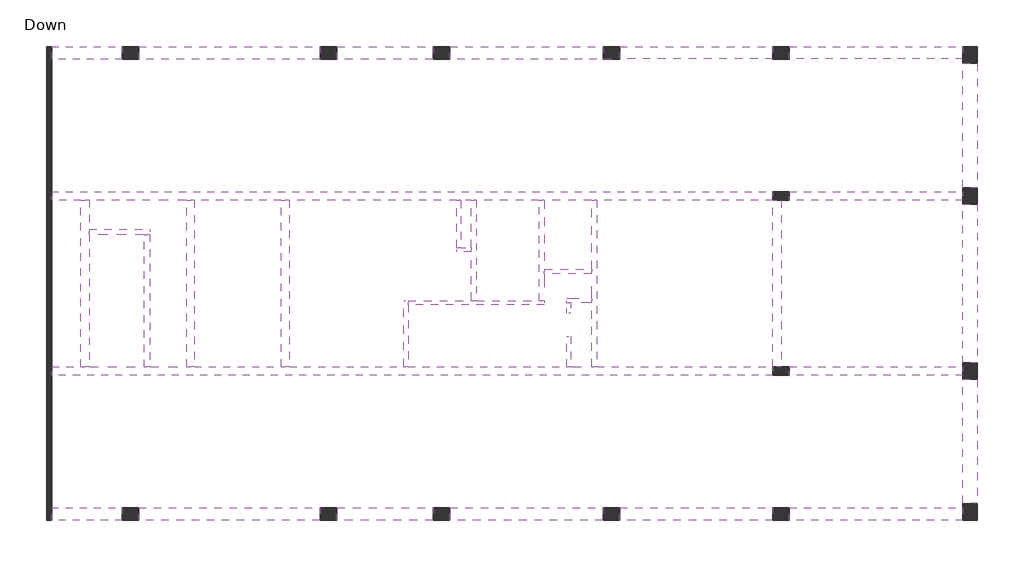
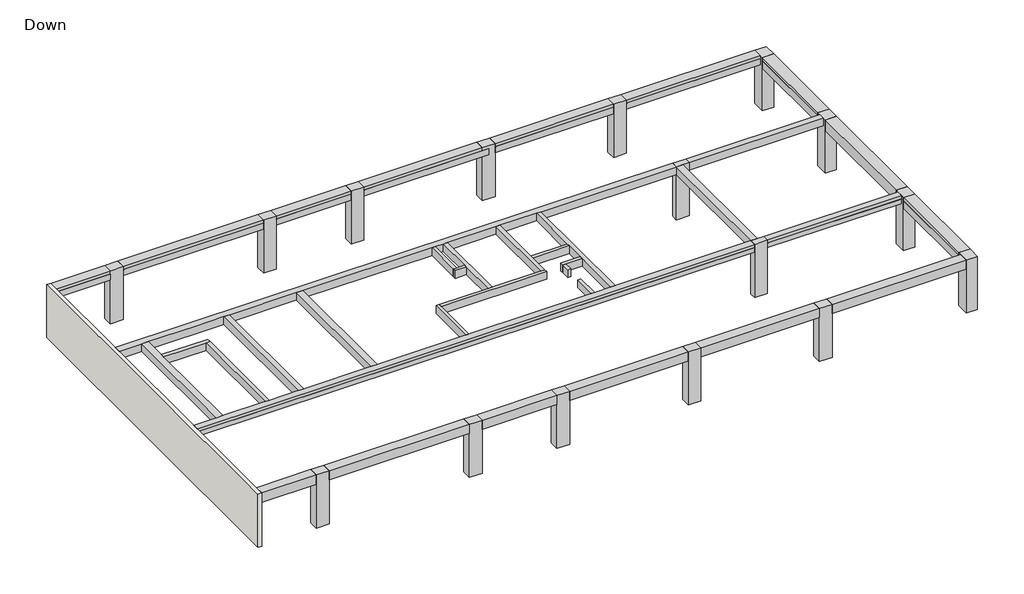
# One storey: 36 beams, 16 columns, 1 wall.
"""IFC4 building model written with IfcOpenShell, lengths in millimetres."""

from ifc_helpers import new_model, si_unit, frame, origin, place, context, project, spatial, polyline, outline, extrude, faceted_brep, element, save

model = new_model("IFC4")

# Units and contexts
model_context = context("Model", 3, world=origin())
ifc_project = project(units=[si_unit("LENGTHUNIT", "METRE", prefix="MILLI")], contexts=[model_context])

# Site, building, storey
site = spatial("IfcSite", under=ifc_project)
building = spatial("IfcBuilding", under=site)
storey = spatial("IfcBuildingStorey", under=building, Name="Down", Elevation=0.0)

# Beams
placement = place(None, origin())
element("IfcBeam", 1, ObjectType="Concrete Rectengular Beam : 20/50", at=placement, inside=storey, context=model_context, shape_type="Brep", body=[
    faceted_brep([(-13392.6687444, -4379.553058, 3500.0), (-13192.6687444, -4379.553058, 3500.0), (-13192.6687444, -1379.553058, 3500.0), (-13192.6687444, -1179.553058, 3500.0), (-13392.6687444, -1179.553058, 3500.0), (-13192.6687444, -4379.553058, 3300.0), (-13192.6687444, -4379.553058, 3000.0), (-13192.6687444, -1379.553058, 3000.0), (-13192.6687444, -1179.553058, 3000.0), (-13192.6687444, -1179.553058, 3300.0), (-13392.6687444, -4379.553058, 3000.0), (-13392.6687444, -1179.553058, 3000.0), (-13392.6687444, -1179.553058, 3300.0), (-13392.6687444, -4379.553058, 3300.0)], [[[0, 1, 2, 3, 4]], [[1, 5, 6, 7, 8, 9, 3, 2]], [[6, 10, 11, 8, 7]], [[0, 4, 12, 11, 10, 13]], [[1, 0, 13, 10, 6, 5]], [[4, 3, 9, 8, 11, 12]]]),
])
element("IfcBeam", 2, ObjectType="Concrete Rectengular Beam : 20/50", at=placement, inside=storey, context=model_context, shape_type="Brep", body=[
    faceted_brep([(-13192.6687444, -1179.553058, 3500.0), (-13192.6687444, -1379.553058, 3500.0), (-6622.8724137, -1379.553058, 3500.0), (-6622.8724137, -1179.553058, 3500.0), (-6872.8724137, -1179.553058, 3500.0), (-9902.8742387, -1179.553058, 3500.0), (-10152.8742387, -1179.553058, 3500.0), (-13192.6687444, -1379.553058, 3300.0), (-13192.6687444, -1379.553058, 3000.0), (-6622.8724137, -1379.553058, 3000.0), (-6622.8724137, -1379.553058, 3300.0), (-13192.6687444, -1179.553058, 3000.0), (-10152.8742387, -1179.553058, 3000.0), (-9902.8742387, -1179.553058, 3000.0), (-6872.8724137, -1179.553058, 3000.0), (-6622.8724137, -1179.553058, 3000.0), (-13192.6687444, -1179.553058, 3300.0), (-6622.8724137, -1179.553058, 3300.0)], [[[0, 1, 2, 3, 4, 5, 6]], [[2, 1, 7, 8, 9, 10]], [[8, 11, 12, 13, 14, 15, 9]], [[15, 14, 13, 12, 11, 16, 0, 6, 5, 4, 3, 17]], [[1, 0, 16, 11, 8, 7]], [[3, 2, 10, 9, 15, 17]]]),
])
element("IfcBeam", 3, ObjectType="Concrete Rectengular Beam : 20/50", at=placement, inside=storey, context=model_context, shape_type="Brep", body=[
    faceted_brep([(-10152.8742387, 1160.4573545, 3500.0), (-10152.8742387, 1360.4573545, 3500.0), (-10647.8742387, 1360.4573545, 3500.0), (-10847.8742387, 1360.4573545, 3500.0), (-10847.8742387, 1160.4573545, 3500.0), (-10152.8742387, 1360.4573545, 3300.0), (-10152.8742387, 1360.4573545, 3000.0), (-10647.8742387, 1360.4573545, 3000.0), (-10847.8742387, 1360.4573545, 3000.0), (-10847.8742387, 1360.4573545, 3300.0), (-10152.8742387, 1160.4573545, 3000.0), (-10847.8742387, 1160.4573545, 3000.0), (-10847.8742387, 1160.4573545, 3300.0), (-10152.8742387, 1160.4573545, 3300.0)], [[[0, 1, 2, 3, 4]], [[1, 5, 6, 7, 8, 9, 3, 2]], [[6, 10, 11, 8, 7]], [[0, 4, 12, 11, 10, 13]], [[1, 0, 13, 10, 6, 5]], [[4, 3, 9, 8, 11, 12]]]),
])
element("IfcBeam", 4, ObjectType="Concrete Rectengular Beam : 20/50", at=placement, inside=storey, context=model_context, shape_type="Brep", body=[
    faceted_brep([(-10847.8742387, 1360.4573545, 3500.0), (-10647.8742387, 1360.4573545, 3500.0), (-10647.8742387, 3660.4573545, 3500.0), (-10847.8742387, 3660.4573545, 3500.0), (-10647.8742387, 1360.4573545, 3300.0), (-10647.8742387, 1360.4573545, 3000.0), (-10647.8742387, 3660.4573545, 3000.0), (-10647.8742387, 3660.4573545, 3300.0), (-10847.8742387, 1360.4573545, 3000.0), (-10847.8742387, 3660.4573545, 3000.0), (-10847.8742387, 3660.4573545, 3300.0), (-10847.8742387, 1360.4573545, 3300.0)], [[[0, 1, 2, 3]], [[1, 4, 5, 6, 7, 2]], [[5, 8, 9, 6]], [[0, 3, 10, 9, 8, 11]], [[1, 0, 11, 8, 5, 4]], [[3, 2, 7, 6, 9, 10]]]),
])
element("IfcBeam", 5, ObjectType="Concrete Rectengular Beam : 20/50", at=placement, inside=storey, context=model_context, shape_type="Brep", body=[
    faceted_brep([(-5552.8714262, -2899.5501705, 3500.0), (-5352.8714262, -2899.5501705, 3500.0), (-5352.8714262, -2899.5501705, 3300.0), (-5352.8714262, -2899.5501705, 3000.0), (-5552.8714262, -2899.5501705, 3000.0), (-5552.8714262, -2899.5501705, 3300.0), (-5552.8714262, -4379.553058, 3500.0), (-5352.8714262, -4379.553058, 3500.0), (-5352.8714262, -4379.553058, 3300.0), (-5352.8714262, -4379.553058, 3000.0), (-5552.8714262, -4379.553058, 3000.0), (-5552.8714262, -4379.553058, 3300.0)], [[[0, 1, 2, 3, 4, 5]], [[1, 0, 6, 7]], [[1, 7, 8, 9, 3, 2]], [[4, 3, 9, 10]], [[6, 0, 5, 4, 10, 11]], [[7, 6, 11, 10, 9, 8]]]),
])
element("IfcBeam", 6, ObjectType="Concrete Rectengular Beam : 20/50", at=placement, inside=storey, context=model_context, shape_type="Brep", body=[
    faceted_brep([(-4337.2434753, -1279.553058, 3500.0), (-4337.2434753, -1079.553058, 3500.0), (-5552.8714262, -1079.553058, 3500.0), (-5552.8714262, -1279.553058, 3500.0), (-5352.8714262, -1279.553058, 3500.0), (-4337.2434753, -1079.553058, 3300.0), (-4337.2434753, -1079.553058, 3000.0), (-5552.8714262, -1079.553058, 3000.0), (-5552.8714262, -1079.553058, 3300.0), (-4337.2434753, -1279.553058, 3000.0), (-5352.8714262, -1279.553058, 3000.0), (-5552.8714262, -1279.553058, 3000.0), (-4337.2434753, -1279.553058, 3300.0), (-5552.8714262, -1279.553058, 3300.0)], [[[0, 1, 2, 3, 4]], [[2, 1, 5, 6, 7, 8]], [[6, 9, 10, 11, 7]], [[11, 10, 9, 12, 0, 4, 3, 13]], [[1, 0, 12, 9, 6, 5]], [[3, 2, 8, 7, 11, 13]]]),
])
element("IfcBeam", 7, ObjectType="Concrete Rectengular Beam : 20/50", at=placement, inside=storey, context=model_context, shape_type="Brep", body=[
    faceted_brep([(-5352.8714262, -1799.553058, 3500.0), (-5552.8714262, -1799.553058, 3500.0), (-5552.8714262, -1799.553058, 3300.0), (-5552.8714262, -1799.553058, 3000.0), (-5352.8714262, -1799.553058, 3000.0), (-5352.8714262, -1799.553058, 3300.0), (-5352.8714262, -1279.553058, 3500.0), (-5552.8714262, -1279.553058, 3500.0), (-5552.8714262, -1279.553058, 3300.0), (-5552.8714262, -1279.553058, 3000.0), (-5352.8714262, -1279.553058, 3000.0), (-5352.8714262, -1279.553058, 3300.0)], [[[0, 1, 2, 3, 4, 5]], [[1, 0, 6, 7]], [[1, 7, 8, 9, 3, 2]], [[4, 3, 9, 10]], [[6, 0, 5, 4, 10, 11]], [[7, 6, 11, 10, 9, 8]]]),
])
element("IfcBeam", 8, ObjectType="Concrete Rectengular Beam : 20/50", at=placement, inside=storey, context=model_context, shape_type="Brep", body=[
    faceted_brep([(-6622.8724137, 320.446942, 3500.0), (-6622.8724137, 120.446942, 3500.0), (-4337.2434753, 120.446942, 3500.0), (-4337.2434753, 320.446942, 3500.0), (-6622.8724137, 320.446942, 3000.0), (-6622.8724137, 320.446942, 3300.0), (-4337.2434753, 320.446942, 3300.0), (-4337.2434753, 320.446942, 3000.0), (-6622.8724137, 120.446942, 3000.0), (-4337.2434753, 120.446942, 3000.0), (-6622.8724137, 120.446942, 3300.0), (-4337.2434753, 120.446942, 3300.0)], [[[0, 1, 2, 3]], [[4, 5, 0, 3, 6, 7]], [[8, 4, 7, 9]], [[1, 10, 8, 9, 11, 2]], [[1, 0, 5, 4, 8, 10]], [[3, 2, 11, 9, 7, 6]]]),
])
element("IfcBeam", 9, ObjectType="Concrete Rectengular Beam : 25/50", at=placement, inside=storey, context=model_context, shape_type="Brep", body=[
    faceted_brep([(-25647.8929888, 2002.2215378, 3500.0), (-25647.8929888, 2252.2215378, 3500.0), (-28552.8929888, 2252.2215378, 3500.0), (-28552.8929888, 2002.2215378, 3500.0), (-25897.8929888, 2002.2215378, 3500.0), (-25647.8929888, 2002.2215378, 3000.0), (-28552.8929888, 2002.2215378, 3000.0), (-25897.8929888, 2002.2215378, 3000.0), (-25647.8929888, 2252.2215378, 3000.0), (-28552.8929888, 2252.2215378, 3000.0)], [[[0, 1, 2, 3, 4]], [[5, 0, 4, 3, 6, 7]], [[8, 5, 7, 6, 9]], [[1, 8, 9, 2]], [[3, 2, 9, 6]], [[1, 0, 5, 8]]]),
])
element("IfcBeam", 10, ObjectType="Concrete Rectengular Beam : 25/50", at=placement, inside=storey, context=model_context, shape_type="Brep", body=[
    faceted_brep([(-25647.8929888, 2002.2215378, 3500.0), (-25897.8929888, 2002.2215378, 3500.0), (-25897.8929888, -4379.553058, 3500.0), (-25647.8929888, -4379.553058, 3500.0), (-25897.8929888, 2002.2215378, 3000.0), (-25897.8929888, -4379.553058, 3000.0), (-25647.8929888, 2002.2215378, 3000.0), (-25647.8929888, -4379.553058, 3000.0), (-25647.8929888, -4379.553058, 3300.0)], [[[0, 1, 2, 3]], [[1, 4, 5, 2]], [[4, 6, 7, 5]], [[6, 0, 3, 8, 7]], [[1, 0, 6, 4]], [[3, 2, 5, 7, 8]]]),
])
element("IfcBeam", 11, ObjectType="Concrete Rectengular Beam : 25/50", at=placement, inside=storey, context=model_context, shape_type="Brep", body=[
    faceted_brep([(-9902.8742387, 3660.4573545, 3500.0), (-10152.8742387, 3660.4573545, 3500.0), (-10152.8742387, 1360.4573545, 3500.0), (-10152.8742387, 1160.4573545, 3500.0), (-10152.8742387, -1179.553058, 3500.0), (-9902.8742387, -1179.553058, 3500.0), (-9902.8742387, 3660.4573545, 3000.0), (-9902.8742387, 3660.4573545, 3300.0), (-9902.8742387, -1179.553058, 3300.0), (-9902.8742387, -1179.553058, 3000.0), (-10152.8742387, 3660.4573545, 3000.0), (-10152.8742387, -1179.553058, 3000.0), (-10152.8742387, 1160.4573545, 3000.0), (-10152.8742387, 1360.4573545, 3000.0), (-10152.8742387, 3660.4573545, 3300.0), (-10152.8742387, -1179.553058, 3300.0)], [[[0, 1, 2, 3, 4, 5]], [[6, 7, 0, 5, 8, 9]], [[10, 6, 9, 11, 12, 13]], [[1, 14, 10, 13, 12, 11, 15, 4, 3, 2]], [[1, 0, 7, 6, 10, 14]], [[5, 4, 15, 11, 9, 8]]]),
])
element("IfcBeam", 12, ObjectType="Concrete Rectengular Beam : 25/50", at=placement, inside=storey, context=model_context, shape_type="Brep", body=[
    faceted_brep([(-6622.8724137, 3660.4573545, 3500.0), (-6872.8724137, 3660.4573545, 3500.0), (-6872.8724137, -1179.553058, 3500.0), (-6622.8724137, -1179.553058, 3500.0), (-6622.8724137, 120.446942, 3500.0), (-6622.8724137, 320.446942, 3500.0), (-6622.8724137, 3660.4573545, 3000.0), (-6622.8724137, 3660.4573545, 3300.0), (-6622.8724137, -1179.553058, 3000.0), (-6622.8724137, 120.446942, 3000.0), (-6622.8724137, 320.446942, 3000.0), (-6872.8724137, 3660.4573545, 3000.0), (-6872.8724137, -1179.553058, 3000.0), (-6872.8724137, 3660.4573545, 3300.0), (-6872.8724137, -1179.553058, 3300.0)], [[[0, 1, 2, 3, 4, 5]], [[6, 7, 0, 5, 4, 3, 8, 9, 10]], [[11, 6, 10, 9, 8, 12]], [[1, 13, 11, 12, 14, 2]], [[1, 0, 7, 6, 11, 13]], [[3, 2, 14, 12, 8]]]),
])
element("IfcBeam", 13, ObjectType="Concrete Rectengular Beam : 25/50", at=placement, inside=storey, context=model_context, shape_type="Brep", body=[
    faceted_brep([(-4087.2434753, 3660.4573545, 3500.0), (-4337.2434753, 3660.4573545, 3500.0), (-4337.2434753, 320.446942, 3500.0), (-4337.2434753, 120.446942, 3500.0), (-4337.2434753, -1079.553058, 3500.0), (-4337.2434753, -1279.553058, 3500.0), (-4337.2434753, -4379.553058, 3500.0), (-4087.2434753, -4379.553058, 3500.0), (-4087.2434753, 3660.4573545, 3000.0), (-4087.2434753, 3660.4573545, 3300.0), (-4087.2434753, -4379.553058, 3300.0), (-4087.2434753, -4379.553058, 3000.0), (-4337.2434753, 3660.4573545, 3000.0), (-4337.2434753, -4379.553058, 3000.0), (-4337.2434753, -1279.553058, 3000.0), (-4337.2434753, -1079.553058, 3000.0), (-4337.2434753, 120.446942, 3000.0), (-4337.2434753, 320.446942, 3000.0), (-4337.2434753, 3660.4573545, 3300.0), (-4337.2434753, -4379.553058, 3300.0)], [[[0, 1, 2, 3, 4, 5, 6, 7]], [[8, 9, 0, 7, 10, 11]], [[12, 8, 11, 13, 14, 15, 16, 17]], [[1, 18, 12, 17, 16, 15, 14, 13, 19, 6, 5, 4, 3, 2]], [[1, 0, 9, 8, 12, 18]], [[7, 6, 19, 13, 11, 10]]]),
])
element("IfcBeam", 14, ObjectType="Concrete Rectengular Beam : 35/50", at=placement, inside=storey, context=model_context, shape_type="Brep", body=[
    faceted_brep([(-23497.8929888, 3660.4573545, 3500.0), (-23847.8929888, 3660.4573545, 3500.0), (-23847.8929888, -4379.553058, 3500.0), (-23497.8929888, -4379.553058, 3500.0), (-23497.8929888, 3660.4573545, 3000.0), (-23497.8929888, 3660.4573545, 3300.0), (-23497.8929888, -4379.553058, 3300.0), (-23497.8929888, -4379.553058, 3000.0), (-23847.8929888, 3660.4573545, 3000.0), (-23847.8929888, -4379.553058, 3000.0), (-23847.8929888, 3660.4573545, 3300.0), (-23847.8929888, -4379.553058, 3300.0)], [[[0, 1, 2, 3]], [[4, 5, 0, 3, 6, 7]], [[8, 4, 7, 9]], [[1, 10, 8, 9, 11, 2]], [[1, 0, 5, 4, 8, 10]], [[3, 2, 11, 9, 7, 6]]]),
])
element("IfcBeam", 15, ObjectType="Concrete Rectengular Beam : 40/50", at=placement, inside=storey, context=model_context, shape_type="Brep", body=[
    faceted_brep([(5187.1402675, 3660.4573545, 3500.0), (13547.1501363, 3660.4573545, 3500.0), (13547.1501363, 4055.4573545, 3500.0), (5187.1402675, 4055.4573545, 3500.0), (13547.1501363, 3660.4573545, 3000.0), (13547.1501363, 3660.4573545, 3300.0), (5187.1402675, 3660.4573545, 3000.0), (5187.1402675, 4060.4573545, 3000.0), (13547.1501363, 4060.4573545, 3000.0), (5187.1402675, 4060.4573545, 3300.0), (13547.1501363, 4060.4573545, 3300.0), (13547.1501363, 4055.4573545, 3300.0), (5187.1402675, 4055.4573545, 3300.0)], [[[0, 1, 2, 3]], [[4, 5, 1, 0, 6]], [[4, 6, 7, 8]], [[8, 7, 9, 10]], [[1, 5, 4, 8, 10, 11, 2]], [[6, 0, 3, 12, 9, 7]], [[12, 11, 10, 9]], [[11, 12, 3, 2]]]),
])
element("IfcBeam", 16, ObjectType="Concrete Rectengular Beam : 40/50", at=placement, inside=storey, context=model_context, shape_type="Brep", body=[
    faceted_brep([(13547.1501363, -4379.553058, 3500.0), (5187.1402675, -4379.553058, 3500.0), (5187.1402675, -4774.553058, 3500.0), (13547.1501363, -4774.553058, 3500.0), (5187.1402675, -4779.553058, 3000.0), (13547.1501363, -4779.553058, 3000.0), (13547.1501363, -4779.553058, 3300.0), (5187.1402675, -4779.553058, 3300.0), (13547.1501363, -4379.553058, 3000.0), (5187.1402675, -4379.553058, 3000.0), (13547.1501363, -4379.553058, 3300.0), (13547.1501363, -4774.553058, 3300.0), (5187.1402675, -4774.553058, 3300.0)], [[[0, 1, 2, 3]], [[4, 5, 6, 7]], [[8, 5, 4, 9]], [[0, 10, 8, 9, 1]], [[8, 10, 0, 3, 11, 6, 5]], [[9, 4, 7, 12, 2, 1]], [[11, 12, 7, 6]], [[12, 11, 3, 2]]]),
])
element("IfcBeam", 17, ObjectType="Concrete Rectengular Beam : 40/50", at=placement, inside=storey, context=model_context, shape_type="Brep", body=[
    faceted_brep([(4387.1402675, 3660.4573545, 3500.0), (4387.1402675, 4055.4573545, 3500.0), (-30362.89442, 4055.4573545, 3500.0), (-30362.89442, 3660.4573545, 3500.0), (-28952.8929888, 3660.4573545, 3500.0), (-28552.8929888, 3660.4573545, 3500.0), (-25647.8929888, 3660.4573545, 3500.0), (-23847.8929888, 3660.4573545, 3500.0), (-23497.8929888, 3660.4573545, 3500.0), (-19308.8564427, 3660.4573545, 3500.0), (-18908.8564427, 3660.4573545, 3500.0), (-10847.8742387, 3660.4573545, 3500.0), (-10647.8742387, 3660.4573545, 3500.0), (-10152.8742387, 3660.4573545, 3500.0), (-9902.8742387, 3660.4573545, 3500.0), (-6872.8724137, 3660.4573545, 3500.0), (-6622.8724137, 3660.4573545, 3500.0), (-4337.2434753, 3660.4573545, 3500.0), (-4087.2434753, 3660.4573545, 3500.0), (4387.1402675, 4060.4573545, 3300.0), (4387.1402675, 4060.4573545, 3000.0), (-30362.89442, 4060.4573545, 3000.0), (-30362.89442, 4060.4573545, 3300.0), (4387.1402675, 3660.4573545, 3000.0), (-4087.2434753, 3660.4573545, 3000.0), (-4337.2434753, 3660.4573545, 3000.0), (-6622.8724137, 3660.4573545, 3000.0), (-6872.8724137, 3660.4573545, 3000.0), (-9902.8742387, 3660.4573545, 3000.0), (-10152.8742387, 3660.4573545, 3000.0), (-10647.8742387, 3660.4573545, 3000.0), (-10847.8742387, 3660.4573545, 3000.0), (-18908.8564427, 3660.4573545, 3000.0), (-19308.8564427, 3660.4573545, 3000.0), (-23497.8929888, 3660.4573545, 3000.0), (-23847.8929888, 3660.4573545, 3000.0), (-28552.8929888, 3660.4573545, 3000.0), (-28952.8929888, 3660.4573545, 3000.0), (-30362.89442, 3660.4573545, 3000.0), (4387.1402675, 3660.4573545, 3300.0), (-30362.89442, 3660.4573545, 3300.0), (4387.1402675, 4055.4573545, 3300.0), (-30362.89442, 4055.4573545, 3300.0)], [[[0, 1, 2, 3, 4, 5, 6, 7, 8, 9, 10, 11, 12, 13, 14, 15, 16, 17, 18]], [[19, 20, 21, 22]], [[20, 23, 24, 25, 26, 27, 28, 29, 30, 31, 32, 33, 34, 35, 36, 37, 38, 21]], [[23, 39, 0, 18, 17, 16, 15, 14, 13, 12, 11, 10, 9, 8, 7, 6, 5, 4, 3, 40, 38, 37, 36, 35, 34, 33, 32, 31, 30, 29, 28, 27, 26, 25, 24]], [[23, 20, 19, 41, 1, 0, 39]], [[41, 19, 22, 42]], [[1, 41, 42, 2]], [[3, 2, 42, 22, 21, 38, 40]]]),
])
element("IfcBeam", 18, ObjectType="Concrete Rectengular Beam : 40/50", at=placement, inside=storey, context=model_context, shape_type="Brep", body=[
    faceted_brep([(4387.1402675, -4774.553058, 3500.0), (4387.1402675, -4379.553058, 3500.0), (-4087.2434753, -4379.553058, 3500.0), (-4337.2434753, -4379.553058, 3500.0), (-5352.8714262, -4379.553058, 3500.0), (-5552.8714262, -4379.553058, 3500.0), (-13192.6687444, -4379.553058, 3500.0), (-13392.6687444, -4379.553058, 3500.0), (-18908.8564427, -4379.553058, 3500.0), (-19308.8564427, -4379.553058, 3500.0), (-23497.8929888, -4379.553058, 3500.0), (-23847.8929888, -4379.553058, 3500.0), (-25647.8929888, -4379.553058, 3500.0), (-25897.8929888, -4379.553058, 3500.0), (-28552.8929888, -4379.553058, 3500.0), (-28952.8929888, -4379.553058, 3500.0), (-30362.89442, -4379.553058, 3500.0), (-30362.89442, -4774.553058, 3500.0), (4387.1402675, -4379.553058, 3300.0), (4387.1402675, -4379.553058, 3000.0), (-4087.2434753, -4379.553058, 3000.0), (-4337.2434753, -4379.553058, 3000.0), (-5352.8714262, -4379.553058, 3000.0), (-5552.8714262, -4379.553058, 3000.0), (-13192.6687444, -4379.553058, 3000.0), (-13392.6687444, -4379.553058, 3000.0), (-18908.8564427, -4379.553058, 3000.0), (-19308.8564427, -4379.553058, 3000.0), (-23497.8929888, -4379.553058, 3000.0), (-23847.8929888, -4379.553058, 3000.0), (-25647.8929888, -4379.553058, 3000.0), (-25897.8929888, -4379.553058, 3000.0), (-28552.8929888, -4379.553058, 3000.0), (-28952.8929888, -4379.553058, 3000.0), (-30362.89442, -4379.553058, 3000.0), (-30362.89442, -4379.553058, 3300.0), (4387.1402675, -4779.553058, 3000.0), (-30362.89442, -4779.553058, 3000.0), (4387.1402675, -4779.553058, 3300.0), (-30362.89442, -4779.553058, 3300.0), (4387.1402675, -4774.553058, 3300.0), (-30362.89442, -4774.553058, 3300.0)], [[[0, 1, 2, 3, 4, 5, 6, 7, 8, 9, 10, 11, 12, 13, 14, 15, 16, 17]], [[1, 18, 19, 20, 21, 22, 23, 24, 25, 26, 27, 28, 29, 30, 31, 32, 33, 34, 35, 16, 15, 14, 13, 12, 11, 10, 9, 8, 7, 6, 5, 4, 3, 2]], [[19, 36, 37, 34, 33, 32, 31, 30, 29, 28, 27, 26, 25, 24, 23, 22, 21, 20]], [[36, 38, 39, 37]], [[19, 18, 1, 0, 40, 38, 36]], [[38, 40, 41, 39]], [[40, 0, 17, 41]], [[17, 16, 35, 34, 37, 39, 41]]]),
])
element("IfcBeam", 19, ObjectType="Concrete Rectengular Beam : 40/50", at=placement, inside=storey, context=model_context, shape_type="Brep", body=[
    faceted_brep([(4387.1402675, -4379.553058, 3500.0), (4787.1402675, -4379.553058, 3500.0), (4787.1402675, 3660.4573545, 3500.0), (4387.1402675, 3660.4573545, 3500.0), (4387.1402675, -4379.553058, 3000.0), (4387.1402675, -4379.553058, 3300.0), (4387.1402675, 3660.4573545, 3300.0), (4387.1402675, 3660.4573545, 3000.0), (4787.1402675, -4379.553058, 3000.0), (4787.1402675, 3660.4573545, 3000.0), (4787.1402675, -4379.553058, 3300.0), (4787.1402675, 3660.4573545, 3300.0)], [[[0, 1, 2, 3]], [[4, 5, 0, 3, 6, 7]], [[8, 4, 7, 9]], [[1, 10, 8, 9, 11, 2]], [[1, 0, 5, 4, 8, 10]], [[3, 2, 11, 9, 7, 6]]]),
])
element("IfcBeam", 20, ObjectType="Concrete Rectengular Beam : 40/50", at=placement, inside=storey, context=model_context, shape_type="Brep", body=[
    faceted_brep([(-28552.8929888, 3660.4573545, 3500.0), (-28952.8929888, 3660.4573545, 3500.0), (-28952.8929888, -4379.553058, 3500.0), (-28552.8929888, -4379.553058, 3500.0), (-28552.8929888, 2002.2215378, 3500.0), (-28552.8929888, 2252.2215378, 3500.0), (-28552.8929888, 3660.4573545, 3000.0), (-28552.8929888, -4379.553058, 3000.0), (-28552.8929888, 2002.2215378, 3000.0), (-28552.8929888, 2252.2215378, 3000.0), (-28952.8929888, 3660.4573545, 3000.0), (-28952.8929888, -4379.553058, 3000.0), (-28952.8929888, 3660.4573545, 3300.0), (-28952.8929888, -4379.553058, 3300.0)], [[[0, 1, 2, 3, 4, 5]], [[6, 0, 5, 4, 3, 7, 8, 9]], [[10, 6, 9, 8, 7, 11]], [[1, 12, 10, 11, 13, 2]], [[1, 0, 6, 10, 12]], [[3, 2, 13, 11, 7]]]),
])
element("IfcBeam", 21, ObjectType="Concrete Rectengular Beam : 40/50", at=placement, inside=storey, context=model_context, shape_type="Brep", body=[
    faceted_brep([(-18908.8564427, 3660.4573545, 3500.0), (-19308.8564427, 3660.4573545, 3500.0), (-19308.8564427, -4379.553058, 3500.0), (-18908.8564427, -4379.553058, 3500.0), (-18908.8564427, 3660.4573545, 3000.0), (-18908.8564427, 3660.4573545, 3300.0), (-18908.8564427, -4379.553058, 3300.0), (-18908.8564427, -4379.553058, 3000.0), (-19308.8564427, 3660.4573545, 3000.0), (-19308.8564427, -4379.553058, 3000.0), (-19308.8564427, 3660.4573545, 3300.0), (-19308.8564427, -4379.553058, 3300.0)], [[[0, 1, 2, 3]], [[4, 5, 0, 3, 6, 7]], [[8, 4, 7, 9]], [[1, 10, 8, 9, 11, 2]], [[1, 0, 5, 4, 8, 10]], [[3, 2, 11, 9, 7, 6]]]),
])
element("IfcBeam", 22, ObjectType="Concrete Rectengular Beam : 60/60", at=placement, inside=storey, context=model_context, shape_type="SweptSolid", body=[
    extrude(outline(polyline([(11060.462042, 2900.0), (10460.462042, 2900.0), (10460.462042, 3300.0), (10462.1426775, 3300.0), (10462.1426775, 3500.0), (11060.462042, 3500.0), (11060.462042, 2900.0)])), frame((5187.1402675, 0.0, 0.0), z_axis=(1.0, 0.0, 0.0), x_axis=(0.0, 1.0, 0.0)), (0.0, 0.0, 1.0), 8360.0098688),
])
element("IfcBeam", 23, ObjectType="Concrete Rectengular Beam : 60/60", at=placement, inside=storey, context=model_context, shape_type="SweptSolid", body=[
    extrude(outline(polyline([(11060.462042, 3500.0), (11060.462042, 2900.0), (10460.462042, 2900.0), (10460.462042, 3300.0), (10462.1426775, 3300.0), (10462.1426775, 3500.0), (11060.462042, 3500.0)])), frame((-2992.8676512, 0.0, 0.0), z_axis=(1.0, 0.0, 0.0), x_axis=(0.0, 1.0, 0.0)), (0.0, 0.0, 1.0), 7380.0079188),
])
element("IfcBeam", 24, ObjectType="Concrete Rectengular Beam : 60/60", at=placement, inside=storey, context=model_context, shape_type="Brep", body=[
    faceted_brep([(-3792.8676512, 11057.1426775, 3500.0), (-11172.875695, 11057.1426775, 3500.0), (-11172.875695, 10462.1426775, 3500.0), (-3792.8676512, 10462.1426775, 3500.0), (-3792.8676512, 11057.1426775, 2900.0), (-11172.875695, 11057.1426775, 2900.0), (-3392.8676512, 10457.1426775, 2900.0), (-11172.875695, 10457.1426775, 2900.0), (-3792.8676512, 10460.462042, 2900.0), (-3392.8676512, 10460.462042, 2900.0), (-3392.8676512, 10457.1426775, 3300.0), (-11172.875695, 10457.1426775, 3300.0), (-3392.8676512, 10460.462042, 3300.0), (-11172.875695, 10462.1426775, 3300.0), (-3792.8676512, 10462.1426775, 3300.0), (-3792.8676512, 10460.462042, 3300.0)], [[[0, 1, 2, 3]], [[0, 4, 5, 1]], [[6, 7, 5, 4, 8, 9]], [[7, 6, 10, 11]], [[6, 9, 12, 10]], [[5, 7, 11, 13, 2, 1]], [[4, 0, 3, 14, 15, 8]], [[9, 8, 15, 12]], [[14, 13, 11, 10, 12, 15]], [[13, 14, 3, 2]]]),
])
element("IfcBeam", 25, ObjectType="Concrete Rectengular Beam : 60/60", at=placement, inside=storey, context=model_context, shape_type="SweptSolid", body=[
    extrude(outline(polyline([(11057.1426775, 3500.0), (11057.1426775, 2900.0), (10457.1426775, 2900.0), (10457.1426775, 3300.0), (10462.1426775, 3300.0), (10462.1426775, 3500.0), (11057.1426775, 3500.0)])), frame((-16632.8798137, 0.0, 0.0), z_axis=(1.0, 0.0, 0.0), x_axis=(0.0, 1.0, 0.0)), (0.0, 0.0, 1.0), 4660.0041188),
])
element("IfcBeam", 26, ObjectType="Concrete Rectengular Beam : 60/60", at=placement, inside=storey, context=model_context, shape_type="SweptSolid", body=[
    extrude(outline(polyline([(11057.1426775, 3500.0), (11057.1426775, 2900.0), (10457.1426775, 2900.0), (10457.1426775, 3300.0), (10462.1426775, 3300.0), (10462.1426775, 3500.0), (11057.1426775, 3500.0)])), frame((-26172.8897575, 0.0, 0.0), z_axis=(1.0, 0.0, 0.0), x_axis=(0.0, 1.0, 0.0)), (0.0, 0.0, 1.0), 8740.0099438),
])
element("IfcBeam", 27, ObjectType="Concrete Rectengular Beam : 60/60", at=placement, inside=storey, context=model_context, shape_type="SweptSolid", body=[
    extrude(outline(polyline([(-11159.5591018, 2900.0), (-11759.5591018, 2900.0), (-11759.5591018, 3500.0), (-11164.5591018, 3500.0), (-11164.5591018, 3300.0), (-11159.5591018, 3300.0), (-11159.5591018, 2900.0)])), frame((-2992.8676512, 0.0, 0.0), z_axis=(1.0, 0.0, 0.0), x_axis=(0.0, 1.0, 0.0)), (0.0, 0.0, 1.0), 7380.0079188),
])
element("IfcBeam", 28, ObjectType="Concrete Rectengular Beam : 60/60", at=placement, inside=storey, context=model_context, shape_type="SweptSolid", body=[
    extrude(outline(polyline([(-11159.5591018, 2900.0), (-11759.5591018, 2900.0), (-11759.5591018, 3500.0), (-11164.5591018, 3500.0), (-11164.5591018, 3300.0), (-11159.5591018, 3300.0), (-11159.5591018, 2900.0)])), frame((-11172.875695, 0.0, 0.0), z_axis=(1.0, 0.0, 0.0), x_axis=(0.0, 1.0, 0.0)), (0.0, 0.0, 1.0), 7380.0080438),
])
element("IfcBeam", 29, ObjectType="Concrete Rectengular Beam : 60/60", at=placement, inside=storey, context=model_context, shape_type="SweptSolid", body=[
    extrude(outline(polyline([(-11159.5591018, 2900.0), (-11759.5591018, 2900.0), (-11759.5591018, 3500.0), (-11164.5591018, 3500.0), (-11164.5591018, 3300.0), (-11159.5591018, 3300.0), (-11159.5591018, 2900.0)])), frame((-16632.8798137, 0.0, 0.0), z_axis=(1.0, 0.0, 0.0), x_axis=(0.0, 1.0, 0.0)), (0.0, 0.0, 1.0), 4660.0041188),
])
element("IfcBeam", 30, ObjectType="Concrete Rectengular Beam : 60/60", at=placement, inside=storey, context=model_context, shape_type="SweptSolid", body=[
    extrude(outline(polyline([(-11159.5591018, 2900.0), (-11759.5591018, 2900.0), (-11759.5591018, 3500.0), (-11164.5591018, 3500.0), (-11164.5591018, 3300.0), (-11159.5591018, 3300.0), (-11159.5591018, 2900.0)])), frame((-26172.8897575, 0.0, 0.0), z_axis=(1.0, 0.0, 0.0), x_axis=(0.0, 1.0, 0.0)), (0.0, 0.0, 1.0), 8740.0099438),
])
element("IfcBeam", 31, ObjectType="Concrete Rectengular Beam : 60/60", at=placement, inside=storey, context=model_context, shape_type="SweptSolid", body=[
    extrude(outline(polyline([(-11759.5591018, 2900.0), (-11759.5591018, 3500.0), (-11164.5591018, 3500.0), (-11164.5591018, 3300.0), (-11159.5591018, 3300.0), (-11159.5591018, 2900.0), (-11759.5591018, 2900.0)])), frame((5187.1402675, 0.0, 0.0), z_axis=(1.0, 0.0, 0.0), x_axis=(0.0, 1.0, 0.0)), (0.0, 0.0, 1.0), 8360.0098688),
])
element("IfcBeam", 32, ObjectType="Concrete Rectengular Beam : 60/60", at=placement, inside=storey, context=model_context, shape_type="SweptSolid", body=[
    extrude(outline(polyline([(-11759.5591018, 3500.0), (-11164.5591018, 3500.0), (-11164.5591018, 3300.0), (-11159.5591018, 3300.0), (-11159.5591018, 2900.0), (-11759.5591018, 2900.0), (-11759.5591018, 3500.0)])), frame((-30362.89442, 0.0, 0.0), z_axis=(1.0, 0.0, 0.0), x_axis=(0.0, 1.0, 0.0)), (0.0, 0.0, 1.0), 3390.0046625),
])
element("IfcBeam", 33, ObjectType="Concrete Rectengular Beam : 60/60", at=placement, inside=storey, context=model_context, shape_type="SweptSolid", body=[
    extrude(outline(polyline([(10462.1426775, 3500.0), (11057.1426775, 3500.0), (11057.1426775, 2900.0), (10457.1426775, 2900.0), (10457.1426775, 3300.0), (10462.1426775, 3300.0), (10462.1426775, 3500.0)])), frame((-30362.89442, 0.0, 0.0), z_axis=(1.0, 0.0, 0.0), x_axis=(0.0, 1.0, 0.0)), (0.0, 0.0, 1.0), 3390.0046625),
])
element("IfcBeam", 34, ObjectType="Concrete Rectengular Beam : 70/70", at=placement, inside=storey, context=model_context, shape_type="SweptSolid", body=[
    extrude(outline(polyline([(2800.0, 13547.1501363), (2800.0, 14247.1501363), (3500.0, 14247.1501363), (3500.0, 13552.1501363), (3300.0, 13552.1501363), (3300.0, 13547.1501363), (2800.0, 13547.1501363)])), frame((0.0, 4260.456417, 0.0), z_axis=(0.0, 1.0, 0.0), x_axis=(0.0, 0.0, 1.0)), (0.0, 0.0, 1.0), 6000.005625),
])
element("IfcBeam", 35, ObjectType="Concrete Rectengular Beam : 70/70", at=placement, inside=storey, context=model_context, shape_type="SweptSolid", body=[
    extrude(outline(polyline([(13547.1501363, 3460.456417), (14247.1501363, 3460.456417), (14247.1501363, -4179.5501205), (13547.1501363, -4179.5501205), (13547.1501363, 3460.456417)])), frame((0.0, 0.0, 2800.0), z_axis=(0.0, 0.0, 1.0), x_axis=(1.0, 0.0, 0.0)), (0.0, 0.0, 1.0), 700.0),
])
element("IfcBeam", 36, ObjectType="Concrete Rectengular Beam : 70/70", at=placement, inside=storey, context=model_context, shape_type="SweptSolid", body=[
    extrude(outline(polyline([(2800.0, 13547.1501363), (2800.0, 14247.1501363), (3500.0, 14247.1501363), (3500.0, 13552.10558), (3300.0, 13552.10558), (3300.0, 13547.1501363), (2800.0, 13547.1501363)])), frame((0.0, -10959.5591018, 0.0), z_axis=(0.0, 1.0, 0.0), x_axis=(0.0, 0.0, 1.0)), (0.0, 0.0, 1.0), 5980.0089813),
])

# Columns
element("IfcColumn", 37, ObjectType="Concrete Rectengular Column : 40/80", at=placement, inside=storey, context=model_context, shape_type="Brep", body=[
    faceted_brep([(4387.1402675, -4379.553058, 0.0), (5187.1402675, -4379.553058, 0.0), (5187.1402675, -4779.553058, 0.0), (4387.1402675, -4779.553058, 0.0), (4387.1402675, -4379.553058, 3500.0), (4787.1402675, -4379.553058, 3500.0), (5187.1402675, -4379.553058, 3500.0), (5187.1402675, -4774.553058, 3500.0), (5187.1402675, -4779.553058, 3500.0), (5187.1402675, -4779.553058, 3300.0), (4387.1402675, -4779.553058, 3500.0), (4387.1402675, -4779.553058, 3300.0), (4387.1402675, -4774.553058, 3500.0)], [[[0, 1, 2, 3]], [[4, 5, 6, 1, 0]], [[6, 7, 8, 9, 2, 1]], [[8, 10, 11, 3, 2, 9]], [[10, 12, 4, 0, 3, 11]], [[4, 12, 10, 8, 7, 6, 5]]]),
])
element("IfcColumn", 38, ObjectType="Concrete Rectengular Column : 40/80", at=placement, inside=storey, context=model_context, shape_type="Brep", body=[
    faceted_brep([(4387.1402675, 4060.4573545, 0.0), (5187.1402675, 4060.4573545, 0.0), (5187.1402675, 3660.4573545, 0.0), (4387.1402675, 3660.4573545, 0.0), (4387.1402675, 4060.4573545, 3500.0), (5187.1402675, 4060.4573545, 3500.0), (5187.1402675, 4060.4573545, 3300.0), (4387.1402675, 4060.4573545, 3000.0), (4387.1402675, 4060.4573545, 3300.0), (5187.1402675, 4055.4573545, 3500.0), (5187.1402675, 3660.4573545, 3500.0), (4787.1402675, 3660.4573545, 3500.0), (4387.1402675, 3660.4573545, 3500.0), (4387.1402675, 3660.4573545, 3000.0), (4387.1402675, 4055.4573545, 3500.0)], [[[0, 1, 2, 3]], [[4, 5, 6, 1, 0, 7, 8]], [[5, 9, 10, 2, 1, 6]], [[10, 11, 12, 13, 3, 2]], [[12, 14, 4, 8, 7, 0, 3, 13]], [[4, 14, 12, 11, 10, 9, 5]]]),
])
element("IfcColumn", 39, ObjectType="Concrete Rectengular Column : 60/80", at=placement, inside=storey, context=model_context, shape_type="Brep", body=[
    faceted_brep([(4387.1402675, -11159.5591018, 0.0), (5187.1402675, -11159.5591018, 0.0), (5187.1402675, -11759.5591018, 0.0), (4387.1402675, -11759.5591018, 0.0), (4387.1402675, -11159.5591018, 3500.0), (5187.1402675, -11159.5591018, 3500.0), (5187.1402675, -11159.5591018, 3300.0), (4387.1402675, -11159.5591018, 3300.0), (5187.1402675, -11164.5591018, 3500.0), (5187.1402675, -11759.5591018, 3500.0), (4387.1402675, -11759.5591018, 3500.0), (4387.1402675, -11164.5591018, 3500.0)], [[[0, 1, 2, 3]], [[4, 5, 6, 1, 0, 7]], [[5, 8, 9, 2, 1, 6]], [[9, 10, 3, 2]], [[10, 11, 4, 7, 0, 3]], [[4, 11, 10, 9, 8, 5]]]),
])
element("IfcColumn", 40, ObjectType="Concrete Rectengular Column : 60/80", at=placement, inside=storey, context=model_context, shape_type="Brep", body=[
    faceted_brep([(-3792.8676512, -11159.5591018, 0.0), (-2992.8676512, -11159.5591018, 0.0), (-2992.8676512, -11759.5591018, 0.0), (-3792.8676512, -11759.5591018, 0.0), (-3792.8676512, -11159.5591018, 3500.0), (-2992.8676512, -11159.5591018, 3500.0), (-2992.8676512, -11159.5591018, 3300.0), (-3792.8676512, -11159.5591018, 3300.0), (-2992.8676512, -11164.5591018, 3500.0), (-2992.8676512, -11759.5591018, 3500.0), (-3792.8676512, -11759.5591018, 3500.0), (-3792.8676512, -11164.5591018, 3500.0)], [[[0, 1, 2, 3]], [[4, 5, 6, 1, 0, 7]], [[5, 8, 9, 2, 1, 6]], [[9, 10, 3, 2]], [[10, 11, 4, 7, 0, 3]], [[4, 11, 10, 9, 8, 5]]]),
])
element("IfcColumn", 41, ObjectType="Concrete Rectengular Column : 60/80", at=placement, inside=storey, context=model_context, shape_type="Brep", body=[
    faceted_brep([(-11972.875695, -11159.5591018, 0.0), (-11172.875695, -11159.5591018, 0.0), (-11172.875695, -11759.5591018, 0.0), (-11972.875695, -11759.5591018, 0.0), (-11972.875695, -11159.5591018, 3500.0), (-11172.875695, -11159.5591018, 3500.0), (-11172.875695, -11159.5591018, 3300.0), (-11972.875695, -11159.5591018, 3300.0), (-11172.875695, -11164.5591018, 3500.0), (-11172.875695, -11759.5591018, 3500.0), (-11972.875695, -11759.5591018, 3500.0), (-11972.875695, -11164.5591018, 3500.0)], [[[0, 1, 2, 3]], [[4, 5, 6, 1, 0, 7]], [[5, 8, 9, 2, 1, 6]], [[9, 10, 3, 2]], [[10, 11, 4, 7, 0, 3]], [[4, 11, 10, 9, 8, 5]]]),
])
element("IfcColumn", 42, ObjectType="Concrete Rectengular Column : 60/80", at=placement, inside=storey, context=model_context, shape_type="Brep", body=[
    faceted_brep([(-17432.8798137, -11159.5591018, 0.0), (-16632.8798137, -11159.5591018, 0.0), (-16632.8798137, -11759.5591018, 0.0), (-17432.8798137, -11759.5591018, 0.0), (-17432.8798137, -11159.5591018, 3500.0), (-16632.8798137, -11159.5591018, 3500.0), (-16632.8798137, -11159.5591018, 3300.0), (-17432.8798137, -11159.5591018, 3300.0), (-16632.8798137, -11164.5591018, 3500.0), (-16632.8798137, -11759.5591018, 3500.0), (-17432.8798137, -11759.5591018, 3500.0), (-17432.8798137, -11164.5591018, 3500.0)], [[[0, 1, 2, 3]], [[4, 5, 6, 1, 0, 7]], [[5, 8, 9, 2, 1, 6]], [[9, 10, 3, 2]], [[10, 11, 4, 7, 0, 3]], [[4, 11, 10, 9, 8, 5]]]),
])
element("IfcColumn", 43, ObjectType="Concrete Rectengular Column : 60/80", at=placement, inside=storey, context=model_context, shape_type="Brep", body=[
    faceted_brep([(-26972.8897575, -11159.5591018, 0.0), (-26172.8897575, -11159.5591018, 0.0), (-26172.8897575, -11759.5591018, 0.0), (-26972.8897575, -11759.5591018, 0.0), (-26972.8897575, -11159.5591018, 3500.0), (-26172.8897575, -11159.5591018, 3500.0), (-26172.8897575, -11159.5591018, 3300.0), (-26972.8897575, -11159.5591018, 3300.0), (-26172.8897575, -11164.5591018, 3500.0), (-26172.8897575, -11759.5591018, 3500.0), (-26972.8897575, -11759.5591018, 3500.0), (-26972.8897575, -11164.5591018, 3500.0)], [[[0, 1, 2, 3]], [[4, 5, 6, 1, 0, 7]], [[5, 8, 9, 2, 1, 6]], [[9, 10, 3, 2]], [[10, 11, 4, 7, 0, 3]], [[4, 11, 10, 9, 8, 5]]]),
])
element("IfcColumn", 44, ObjectType="Concrete Rectengular Column : 60/80", at=placement, inside=storey, context=model_context, shape_type="Brep", body=[
    faceted_brep([(-26972.8897575, 11057.1426775, 0.0), (-26172.8897575, 11057.1426775, 0.0), (-26172.8897575, 10457.1426775, 0.0), (-26972.8897575, 10457.1426775, 0.0), (-26972.8897575, 11057.1426775, 3500.0), (-26172.8897575, 11057.1426775, 3500.0), (-26172.8897575, 10462.1426775, 3500.0), (-26172.8897575, 10457.1426775, 3500.0), (-26172.8897575, 10457.1426775, 3300.0), (-26972.8897575, 10457.1426775, 3500.0), (-26972.8897575, 10457.1426775, 3300.0), (-26972.8897575, 10462.1426775, 3500.0)], [[[0, 1, 2, 3]], [[4, 5, 1, 0]], [[5, 6, 7, 8, 2, 1]], [[7, 9, 10, 3, 2, 8]], [[9, 11, 4, 0, 3, 10]], [[4, 11, 9, 7, 6, 5]]]),
])
element("IfcColumn", 45, ObjectType="Concrete Rectengular Column : 60/80", at=placement, inside=storey, context=model_context, shape_type="Brep", body=[
    faceted_brep([(-17432.8798137, 11057.1426775, 0.0), (-16632.8798137, 11057.1426775, 0.0), (-16632.8798137, 10457.1426775, 0.0), (-17432.8798137, 10457.1426775, 0.0), (-17432.8798137, 11057.1426775, 3500.0), (-16632.8798137, 11057.1426775, 3500.0), (-16632.8798137, 10462.1426775, 3500.0), (-16632.8798137, 10457.1426775, 3500.0), (-16632.8798137, 10457.1426775, 3300.0), (-17432.8798137, 10457.1426775, 3500.0), (-17432.8798137, 10457.1426775, 3300.0), (-17432.8798137, 10462.1426775, 3500.0)], [[[0, 1, 2, 3]], [[4, 5, 1, 0]], [[5, 6, 7, 8, 2, 1]], [[7, 9, 10, 3, 2, 8]], [[9, 11, 4, 0, 3, 10]], [[4, 11, 9, 7, 6, 5]]]),
])
element("IfcColumn", 46, ObjectType="Concrete Rectengular Column : 60/80", at=placement, inside=storey, context=model_context, shape_type="Brep", body=[
    faceted_brep([(-11972.875695, 11057.1426775, 0.0), (-11172.875695, 11057.1426775, 0.0), (-11172.875695, 10457.1426775, 0.0), (-11972.875695, 10457.1426775, 0.0), (-11972.875695, 11057.1426775, 3500.0), (-11172.875695, 11057.1426775, 3500.0), (-11172.875695, 10462.1426775, 3500.0), (-11172.875695, 10457.1426775, 3500.0), (-11172.875695, 10457.1426775, 3300.0), (-11972.875695, 10457.1426775, 3500.0), (-11972.875695, 10457.1426775, 3300.0), (-11972.875695, 10462.1426775, 3500.0)], [[[0, 1, 2, 3]], [[4, 5, 1, 0]], [[5, 6, 7, 8, 2, 1]], [[7, 9, 10, 3, 2, 8]], [[9, 11, 4, 0, 3, 10]], [[4, 11, 9, 7, 6, 5]]]),
])
element("IfcColumn", 47, ObjectType="Concrete Rectengular Column : 60/80", at=placement, inside=storey, context=model_context, shape_type="Brep", body=[
    faceted_brep([(-3792.8676512, 11060.462042, 0.0), (-2992.8676512, 11060.462042, 0.0), (-2992.8676512, 10460.462042, 0.0), (-3792.8676512, 10460.462042, 0.0), (-3792.8676512, 11060.462042, 3500.0), (-2992.8676512, 11060.462042, 3500.0), (-2992.8676512, 10462.1426775, 3500.0), (-2992.8676512, 10460.462042, 3500.0), (-2992.8676512, 10460.462042, 3300.0), (-3792.8676512, 10460.462042, 3500.0), (-3792.8676512, 10460.462042, 3300.0), (-3792.8676512, 10462.1426775, 3500.0)], [[[0, 1, 2, 3]], [[4, 5, 1, 0]], [[5, 6, 7, 8, 2, 1]], [[7, 9, 10, 3, 2, 8]], [[9, 11, 4, 0, 3, 10]], [[4, 11, 9, 7, 6, 5]]]),
])
element("IfcColumn", 48, ObjectType="Concrete Rectengular Column : 60/80", at=placement, inside=storey, context=model_context, shape_type="Brep", body=[
    faceted_brep([(4387.1402675, 11060.462042, 0.0), (5187.1402675, 11060.462042, 0.0), (5187.1402675, 10460.462042, 0.0), (4387.1402675, 10460.462042, 0.0), (4387.1402675, 11060.462042, 3500.0), (5187.1402675, 11060.462042, 3500.0), (5187.1402675, 10462.1426775, 3500.0), (5187.1402675, 10460.462042, 3500.0), (5187.1402675, 10460.462042, 3300.0), (4387.1402675, 10460.462042, 3500.0), (4387.1402675, 10460.462042, 3300.0), (4387.1402675, 10462.1426775, 3500.0)], [[[0, 1, 2, 3]], [[4, 5, 1, 0]], [[5, 6, 7, 8, 2, 1]], [[7, 9, 10, 3, 2, 8]], [[9, 11, 4, 0, 3, 10]], [[4, 11, 9, 7, 6, 5]]]),
])
element("IfcColumn", 49, ObjectType="Concrete Rectengular Column : 80/70", at=placement, inside=storey, context=model_context, shape_type="Brep", body=[
    faceted_brep([(13547.1501363, 11060.462042, 0.0), (14247.1501363, 11060.462042, 0.0), (14247.1501363, 10260.462042, 0.0), (13547.1501363, 10260.462042, 0.0), (13547.1501363, 11060.462042, 3500.0), (14247.1501363, 11060.462042, 3500.0), (14247.1501363, 10260.462042, 3500.0), (13552.1501363, 10260.462042, 3500.0), (13547.1501363, 10260.462042, 3500.0), (13547.1501363, 10260.462042, 3300.0), (13547.1501363, 10462.1426775, 3500.0)], [[[0, 1, 2, 3]], [[4, 5, 1, 0]], [[5, 6, 2, 1]], [[6, 7, 8, 9, 3, 2]], [[8, 10, 4, 0, 3, 9]], [[4, 10, 8, 7, 6, 5]]]),
])
element("IfcColumn", 50, ObjectType="Concrete Rectengular Column : 80/70", at=placement, inside=storey, context=model_context, shape_type="Brep", body=[
    faceted_brep([(13547.1501363, 4260.456417, 0.0), (14247.1501363, 4260.456417, 0.0), (14247.1501363, 3460.456417, 0.0), (13547.1501363, 3460.456417, 0.0), (13547.1501363, 4260.456417, 3500.0), (13552.1501363, 4260.456417, 3500.0), (14247.1501363, 4260.456417, 3500.0), (13547.1501363, 4260.456417, 3300.0), (14247.1501363, 3460.456417, 3500.0), (13547.1501363, 3460.456417, 3500.0), (13547.1501363, 3660.4573545, 3500.0), (13547.1501363, 4055.4573545, 3500.0)], [[[0, 1, 2, 3]], [[4, 5, 6, 1, 0, 7]], [[6, 8, 2, 1]], [[8, 9, 3, 2]], [[9, 10, 11, 4, 7, 0, 3]], [[4, 11, 10, 9, 8, 6, 5]]]),
])
element("IfcColumn", 51, ObjectType="Concrete Rectengular Column : 80/70", at=placement, inside=storey, context=model_context, shape_type="Brep", body=[
    faceted_brep([(13547.1501363, -4179.5501205, 0.0), (14247.1501363, -4179.5501205, 0.0), (14247.1501363, -4979.5501205, 0.0), (13547.1501363, -4979.5501205, 0.0), (13547.1501363, -4179.5501205, 3500.0), (14247.1501363, -4179.5501205, 3500.0), (14247.1501363, -4979.5501205, 3500.0), (13552.10558, -4979.5501205, 3500.0), (13547.1501363, -4979.5501205, 3500.0), (13547.1501363, -4979.5501205, 3300.0), (13547.1501363, -4774.553058, 3500.0), (13547.1501363, -4379.553058, 3500.0)], [[[0, 1, 2, 3]], [[4, 5, 1, 0]], [[5, 6, 2, 1]], [[6, 7, 8, 9, 3, 2]], [[8, 10, 11, 4, 0, 3, 9]], [[4, 11, 10, 8, 7, 6, 5]]]),
])
element("IfcColumn", 52, ObjectType="Concrete Rectengular Column : 80/70", at=placement, inside=storey, context=model_context, shape_type="Brep", body=[
    faceted_brep([(13547.1501363, -10959.5591018, 0.0), (14247.1501363, -10959.5591018, 0.0), (14247.1501363, -11759.5591018, 0.0), (13547.1501363, -11759.5591018, 0.0), (13547.1501363, -10959.5591018, 3500.0), (13552.10558, -10959.5591018, 3500.0), (14247.1501363, -10959.5591018, 3500.0), (13547.1501363, -10959.5591018, 3300.0), (14247.1501363, -11759.5591018, 3500.0), (13547.1501363, -11759.5591018, 3500.0), (13547.1501363, -11164.5591018, 3500.0)], [[[0, 1, 2, 3]], [[4, 5, 6, 1, 0, 7]], [[6, 8, 2, 1]], [[8, 9, 3, 2]], [[9, 10, 4, 7, 0, 3]], [[4, 10, 9, 8, 6, 5]]]),
])

# Wall
element("IfcWall", 53, ObjectType="25", at=placement, inside=storey, context=model_context, shape_type="Brep", body=[
    faceted_brep([(-30362.89442, -11759.5591018, 0.0), (-30362.89442, 11057.1426775, 0.0), (-30362.89442, 11057.1426775, 2900.0), (-30362.89442, 11057.1426775, 3500.0), (-30362.89442, 10462.1426775, 3500.0), (-30362.89442, 4055.4573545, 3500.0), (-30362.89442, 3660.4573545, 3500.0), (-30362.89442, -4379.553058, 3500.0), (-30362.89442, -4774.553058, 3500.0), (-30362.89442, -11164.5591018, 3500.0), (-30362.89442, -11759.5591018, 3500.0), (-30362.89442, -11759.5591018, 2900.0), (-30612.89442, -11759.5591018, 0.0), (-30612.89442, -11759.5591018, 3500.0), (-30612.89442, 11057.1426775, 3500.0), (-30612.89442, 11057.1426775, 0.0)], [[[0, 1, 2, 3, 4, 5, 6, 7, 8, 9, 10, 11]], [[12, 13, 14, 15]], [[1, 0, 12, 15]], [[3, 2, 1, 15, 14]], [[10, 9, 8, 7, 6, 5, 4, 3, 14, 13]], [[0, 11, 10, 13, 12]]]),
])

save(model, "model.ifc")

# Revit data of these elements
# Project information
#   Project Issue Date = "Issue Date"
#   Project Status = "Project Status"
#   Client Name = "לקוח"
#   Project Address = "Enter address here"
#   Project Name = "Project 029"
#   Project Number = "מספר פרויקט"
# Type "Concrete Rectengular Beam : 20/50"
#   Length [instance default] = 152.4 cm
#   b = 20 cm
#   h = 50 cm
#   Structural Material [instance default] = Concrete
#   Assembly Code = ""
# Type "Concrete Rectengular Beam : 25/50"
#   Length [instance default] = 152.4 cm
#   b = 25 cm
#   h = 50 cm
#   Structural Material [instance default] = Concrete
#   Assembly Code = ""
# Type "Concrete Rectengular Beam : 35/50"
#   Length [instance default] = 152.4 cm
#   b = 35 cm
#   h = 50 cm
#   Structural Material [instance default] = Concrete
#   Assembly Code = ""
# Type "Concrete Rectengular Beam : 40/50"
#   Length [instance default] = 152.4 cm
#   b = 40 cm
#   h = 50 cm
#   Structural Material [instance default] = Concrete
#   Assembly Code = ""
# Type "Concrete Rectengular Beam : 60/60"
#   Length [instance default] = 152.4 cm
#   b = 60 cm
#   h = 60 cm
#   Structural Material [instance default] = Concrete
#   Assembly Code = ""
# Type "Concrete Rectengular Beam : 70/70"
#   Length [instance default] = 152.4 cm
#   b = 70 cm
#   h = 70 cm
#   Structural Material [instance default] = Concrete
#   Assembly Code = ""
# Type "Concrete Rectengular Column : 40/80"
#   b = 40 cm
#   h = 80 cm
#   Structural Material [instance default] = Concrete
# Type "Concrete Rectengular Column : 60/80"
#   b = 60 cm
#   h = 80 cm
#   Structural Material [instance default] = Concrete
# Type "Concrete Rectengular Column : 80/70"
#   b = 80 cm
#   h = 70 cm
#   Structural Material [instance default] = Concrete
# Type "25"
#   Layers, outside or top first: 25 cm "Concrete" (function 1)
# Element 1 (IfcBeam, "Concrete Rectengular Beam : 20/50")
#   Comments = ""
#   Mark = "B1"
#   SOFiSTiK_AMG_Comments = ""
#   SOFiSTiK_AMG_Scheduled = yes
#   SOFiSTiK_AMG_Adjusted = yes
#   Structural Material = Concrete
#   Phase Created = New Construction
#   Materials on its faces: "Concrete"
# Element 2 (IfcBeam, "Concrete Rectengular Beam : 20/50")
#   Comments = ""
#   Mark = "B2"
#   SOFiSTiK_AMG_Comments = ""
#   SOFiSTiK_AMG_Scheduled = yes
#   SOFiSTiK_AMG_Adjusted = yes
#   Structural Material = Concrete
#   Phase Created = New Construction
#   Materials on its faces: "Concrete"
# Element 3 (IfcBeam, "Concrete Rectengular Beam : 20/50")
#   Comments = ""
#   Mark = "B3"
#   SOFiSTiK_AMG_Comments = ""
#   SOFiSTiK_AMG_Scheduled = yes
#   SOFiSTiK_AMG_Adjusted = yes
#   Structural Material = Concrete
#   Phase Created = New Construction
#   Materials on its faces: "Concrete"
# Element 4 (IfcBeam, "Concrete Rectengular Beam : 20/50")
#   Comments = ""
#   Mark = "B4"
#   SOFiSTiK_AMG_Comments = ""
#   SOFiSTiK_AMG_Scheduled = yes
#   SOFiSTiK_AMG_Adjusted = yes
#   Structural Material = Concrete
#   Phase Created = New Construction
#   Materials on its faces: "Concrete"
# Element 5 (IfcBeam, "Concrete Rectengular Beam : 20/50")
#   Comments = ""
#   Mark = "B5"
#   SOFiSTiK_AMG_Comments = ""
#   SOFiSTiK_AMG_Scheduled = yes
#   SOFiSTiK_AMG_Adjusted = yes
#   Structural Material = Concrete
#   Phase Created = New Construction
#   Materials on its faces: "Concrete"
# Element 6 (IfcBeam, "Concrete Rectengular Beam : 20/50")
#   Comments = ""
#   Mark = "B6"
#   SOFiSTiK_AMG_Comments = ""
#   SOFiSTiK_AMG_Scheduled = yes
#   SOFiSTiK_AMG_Adjusted = yes
#   Structural Material = Concrete
#   Phase Created = New Construction
#   Materials on its faces: "Concrete"
# Element 7 (IfcBeam, "Concrete Rectengular Beam : 20/50")
#   Comments = ""
#   Mark = "B7"
#   SOFiSTiK_AMG_Comments = ""
#   SOFiSTiK_AMG_Scheduled = yes
#   SOFiSTiK_AMG_Adjusted = yes
#   Structural Material = Concrete
#   Phase Created = New Construction
#   Materials on its faces: "Concrete"
# Element 8 (IfcBeam, "Concrete Rectengular Beam : 20/50")
#   Comments = ""
#   Mark = "B8"
#   SOFiSTiK_AMG_Comments = ""
#   SOFiSTiK_AMG_Scheduled = yes
#   SOFiSTiK_AMG_Adjusted = yes
#   Structural Material = Concrete
#   Phase Created = New Construction
#   Materials on its faces: "Concrete"
# Element 9 (IfcBeam, "Concrete Rectengular Beam : 25/50")
#   Comments = ""
#   Mark = "B9"
#   SOFiSTiK_AMG_Comments = ""
#   SOFiSTiK_AMG_Scheduled = yes
#   SOFiSTiK_AMG_Adjusted = yes
#   Structural Material = Concrete
#   Phase Created = New Construction
#   Materials on its faces: "Concrete"
# Element 10 (IfcBeam, "Concrete Rectengular Beam : 25/50")
#   Comments = ""
#   Mark = "B10"
#   SOFiSTiK_AMG_Comments = ""
#   SOFiSTiK_AMG_Scheduled = yes
#   SOFiSTiK_AMG_Adjusted = yes
#   Structural Material = Concrete
#   Phase Created = New Construction
#   Materials on its faces: "Concrete"
# Element 11 (IfcBeam, "Concrete Rectengular Beam : 25/50")
#   Comments = ""
#   Mark = "B11"
#   SOFiSTiK_AMG_Comments = ""
#   SOFiSTiK_AMG_Scheduled = yes
#   SOFiSTiK_AMG_Adjusted = yes
#   Structural Material = Concrete
#   Phase Created = New Construction
#   Materials on its faces: "Concrete"
# Element 12 (IfcBeam, "Concrete Rectengular Beam : 25/50")
#   Comments = ""
#   Mark = "B12"
#   SOFiSTiK_AMG_Comments = ""
#   SOFiSTiK_AMG_Scheduled = yes
#   SOFiSTiK_AMG_Adjusted = yes
#   Structural Material = Concrete
#   Phase Created = New Construction
#   Materials on its faces: "Concrete"
# Element 13 (IfcBeam, "Concrete Rectengular Beam : 25/50")
#   Comments = ""
#   Mark = "B13"
#   SOFiSTiK_AMG_Comments = ""
#   SOFiSTiK_AMG_Scheduled = yes
#   SOFiSTiK_AMG_Adjusted = yes
#   Structural Material = Concrete
#   Phase Created = New Construction
#   Materials on its faces: "Concrete"
# Element 14 (IfcBeam, "Concrete Rectengular Beam : 35/50")
#   Comments = ""
#   Mark = "B14"
#   SOFiSTiK_AMG_Comments = ""
#   SOFiSTiK_AMG_Scheduled = yes
#   SOFiSTiK_AMG_Adjusted = yes
#   Structural Material = Concrete
#   Phase Created = New Construction
#   Materials on its faces: "Concrete"
# Element 15 (IfcBeam, "Concrete Rectengular Beam : 40/50")
#   Comments = ""
#   Mark = "B15"
#   SOFiSTiK_AMG_Comments = ""
#   SOFiSTiK_AMG_Scheduled = yes
#   SOFiSTiK_AMG_Adjusted = yes
#   Structural Material = Concrete
#   Phase Created = New Construction
#   Materials on its faces: "Concrete"
# Element 16 (IfcBeam, "Concrete Rectengular Beam : 40/50")
#   Comments = ""
#   Mark = "B16"
#   SOFiSTiK_AMG_Comments = ""
#   SOFiSTiK_AMG_Scheduled = yes
#   SOFiSTiK_AMG_Adjusted = yes
#   Structural Material = Concrete
#   Phase Created = New Construction
#   Materials on its faces: "Concrete"
# Element 17 (IfcBeam, "Concrete Rectengular Beam : 40/50")
#   Comments = ""
#   Mark = "B17"
#   SOFiSTiK_AMG_Comments = ""
#   SOFiSTiK_AMG_Scheduled = yes
#   SOFiSTiK_AMG_Adjusted = yes
#   Structural Material = Concrete
#   Phase Created = New Construction
#   Materials on its faces: "Concrete"
# Element 18 (IfcBeam, "Concrete Rectengular Beam : 40/50")
#   Comments = ""
#   Mark = "B18"
#   SOFiSTiK_AMG_Comments = ""
#   SOFiSTiK_AMG_Scheduled = yes
#   SOFiSTiK_AMG_Adjusted = yes
#   Structural Material = Concrete
#   Phase Created = New Construction
#   Materials on its faces: "Concrete"
# Element 19 (IfcBeam, "Concrete Rectengular Beam : 40/50")
#   Comments = ""
#   Mark = "B19"
#   SOFiSTiK_AMG_Comments = ""
#   SOFiSTiK_AMG_Scheduled = yes
#   SOFiSTiK_AMG_Adjusted = yes
#   Structural Material = Concrete
#   Phase Created = New Construction
#   Materials on its faces: "Concrete"
# Element 20 (IfcBeam, "Concrete Rectengular Beam : 40/50")
#   Comments = ""
#   Mark = "B20"
#   SOFiSTiK_AMG_Comments = ""
#   SOFiSTiK_AMG_Scheduled = yes
#   SOFiSTiK_AMG_Adjusted = yes
#   Structural Material = Concrete
#   Phase Created = New Construction
#   Materials on its faces: "Concrete"
# Element 21 (IfcBeam, "Concrete Rectengular Beam : 40/50")
#   Comments = ""
#   Mark = "B21"
#   SOFiSTiK_AMG_Comments = ""
#   SOFiSTiK_AMG_Scheduled = yes
#   SOFiSTiK_AMG_Adjusted = yes
#   Structural Material = Concrete
#   Phase Created = New Construction
#   Materials on its faces: "Concrete"
# Element 22 (IfcBeam, "Concrete Rectengular Beam : 60/60")
#   Comments = ""
#   Mark = "B22"
#   SOFiSTiK_AMG_Comments = ""
#   SOFiSTiK_AMG_Scheduled = yes
#   SOFiSTiK_AMG_Adjusted = yes
#   Structural Material = Concrete
#   Phase Created = New Construction
#   Materials on its faces: "Concrete"
# Element 23 (IfcBeam, "Concrete Rectengular Beam : 60/60")
#   Comments = ""
#   Mark = "B23"
#   SOFiSTiK_AMG_Comments = ""
#   SOFiSTiK_AMG_Scheduled = yes
#   SOFiSTiK_AMG_Adjusted = yes
#   Structural Material = Concrete
#   Phase Created = New Construction
#   Materials on its faces: "Concrete"
# Element 24 (IfcBeam, "Concrete Rectengular Beam : 60/60")
#   Comments = ""
#   Mark = "B24"
#   SOFiSTiK_AMG_Comments = ""
#   SOFiSTiK_AMG_Scheduled = yes
#   SOFiSTiK_AMG_Adjusted = yes
#   Structural Material = Concrete
#   Phase Created = New Construction
#   Materials on its faces: "Concrete"
# Element 25 (IfcBeam, "Concrete Rectengular Beam : 60/60")
#   Comments = ""
#   Mark = "B25"
#   SOFiSTiK_AMG_Comments = ""
#   SOFiSTiK_AMG_Scheduled = yes
#   SOFiSTiK_AMG_Adjusted = yes
#   Structural Material = Concrete
#   Phase Created = New Construction
#   Materials on its faces: "Concrete"
# Element 26 (IfcBeam, "Concrete Rectengular Beam : 60/60")
#   Comments = ""
#   Mark = "B26"
#   SOFiSTiK_AMG_Comments = ""
#   SOFiSTiK_AMG_Scheduled = yes
#   SOFiSTiK_AMG_Adjusted = yes
#   Structural Material = Concrete
#   Phase Created = New Construction
#   Materials on its faces: "Concrete"
# Element 27 (IfcBeam, "Concrete Rectengular Beam : 60/60")
#   Comments = ""
#   Mark = "B27"
#   SOFiSTiK_AMG_Comments = ""
#   SOFiSTiK_AMG_Scheduled = yes
#   SOFiSTiK_AMG_Adjusted = yes
#   Structural Material = Concrete
#   Phase Created = New Construction
#   Materials on its faces: "Concrete"
# Element 28 (IfcBeam, "Concrete Rectengular Beam : 60/60")
#   Comments = ""
#   Mark = "B28"
#   SOFiSTiK_AMG_Comments = ""
#   SOFiSTiK_AMG_Scheduled = yes
#   SOFiSTiK_AMG_Adjusted = yes
#   Structural Material = Concrete
#   Phase Created = New Construction
#   Materials on its faces: "Concrete"
